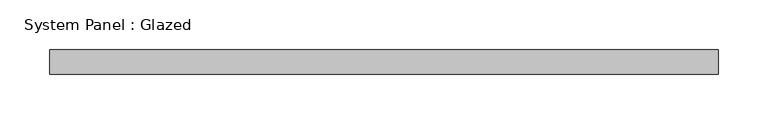
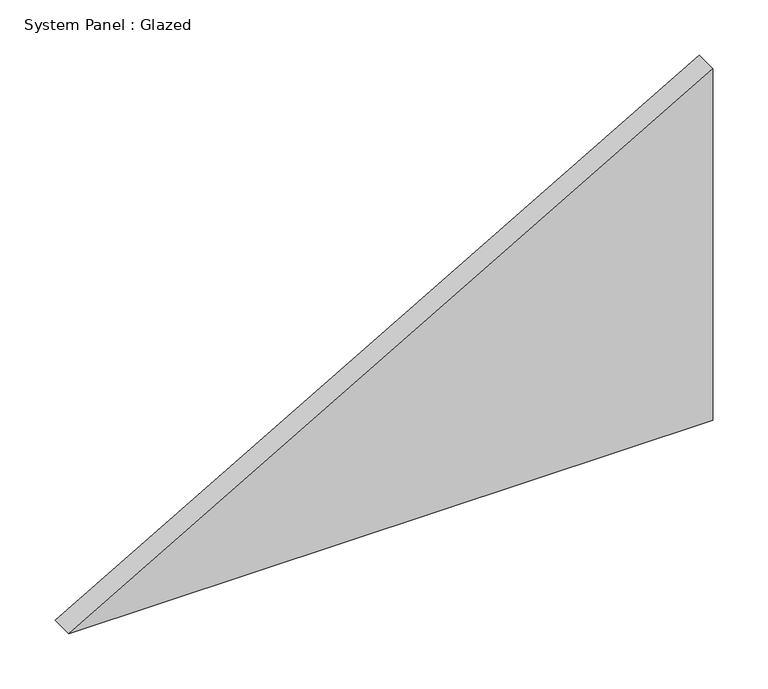
"""IFC4 building model written with IfcOpenShell, lengths in millimetres: plate geometry, System Panel : Glazed."""

from ifc_helpers import new_model, si_unit, frame, origin, place, context, project, spatial, polyline, outline, extrude, source, transform, mapped, element, save


def system_panel_glazed_4ae31ee8(model_context):
    return source(origin(), model_context, "Body", "SweptSolid", [
        extrude(outline(polyline([(0.0, -337.4252157), (0.0, 337.4252157), (389.6250782, 337.4252157), (0.0, -337.4252157)])), frame((0.0, 24.5, 0.0), z_axis=(0.0, 1.0, 0.0), x_axis=(0.0, 0.0, 1.0)), (0.0, 0.0, 1.0), 25.0),
    ])


if __name__ == "__main__":
    model = new_model("IFC4")
    model_context = context("Model", 3, world=origin())
    ifc_project = project(units=[si_unit("LENGTHUNIT", "METRE", prefix="MILLI")], contexts=[model_context])
    site = spatial("IfcSite", under=ifc_project)
    building = spatial("IfcBuilding", under=site)
    placement = place(None, origin())
    system_panel_glazed_shape = system_panel_glazed_4ae31ee8(model_context)
    element("IfcPlate", 1, ObjectType="System Panel : Glazed", at=placement, inside=building, context=model_context, shape_type="MappedRepresentation", body=[
        mapped(system_panel_glazed_shape, transform((0.0, 0.0, 0.0), x_axis=(1.0, 0.0, 0.0), y_axis=(0.0, 1.0, 0.0), z_axis=(0.0, 0.0, 1.0))),
    ])
    save(model, "model.ifc")

# Revit data of these elements
# Type "System Panel : Glazed"
#   Construction Type Id = "GSP4R"
#   Analytic Construction = "1/8 in Pilkington single glazing"
#   Visual Light Transmittance = 0.9
#   Solar Heat Gain Coefficient = 0.86
#   Heat Transfer Coefficient (U) = 6.7069 W/(m²·K)
#   Define Thermal Properties by = 1
# Element 1 (IfcPlate, "System Panel : Glazed")
#   Materials on its faces: "Glass"
# Materials
#   "Glass": class "Glass", colour RGB 0 128 192, transparency 0.75, Description = "Soda Lime Glass", Cost = 0
